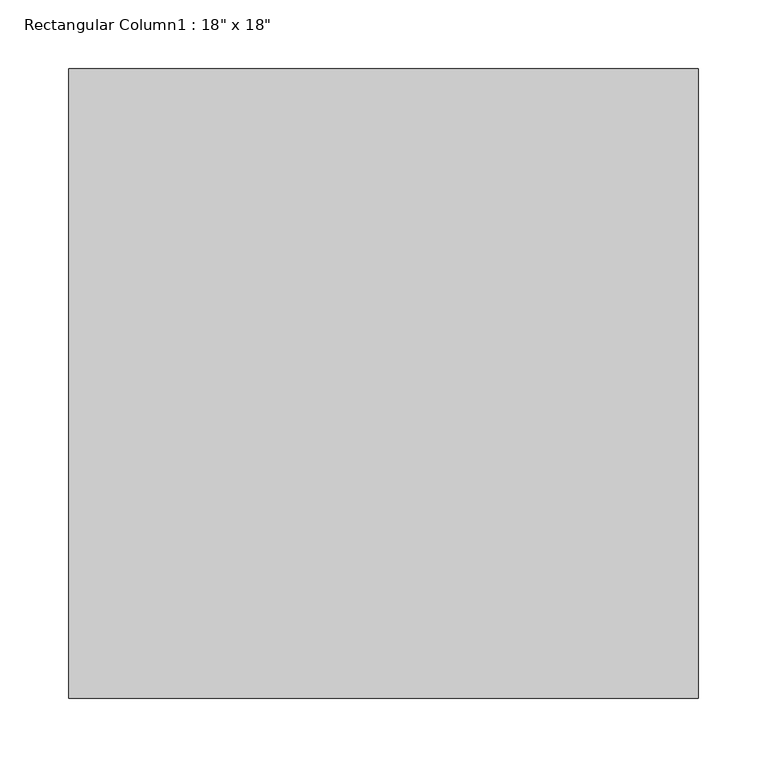
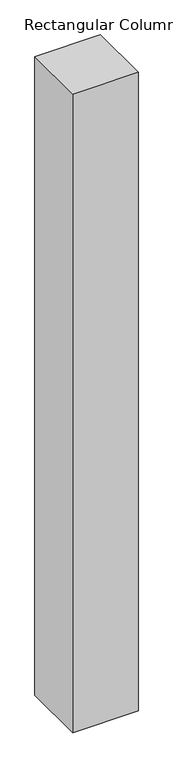
"""IFC4 building model written with IfcOpenShell, lengths in millimetres: column geometry."""

import ifcopenshell
import ifcopenshell.guid

model = None  # the IFC model being written
_history = None  # IfcOwnerHistory: only IFC2X3 demands one
_inside = {}  # id of a spatial element -> (the spatial element, [elements in it])
_under = {}  # id of a project, library or spatial element -> (it, [spatial elements below it])
_declared = {}  # id of a project -> (the project, [libraries it declares])
_typed = {}  # id of a type object -> (the type object, [elements of that type])
_made_of = {}  # id of a material, layer set ... -> (it, [elements and type objects made of it])


def new_model(schema):
    """Start an empty IFC model of exactly this schema.

    Asked for "IFC4X3", IfcOpenShell would pick the latest addendum, in which some entities
    have other attributes; the version numbers below select the first issue.
    IFC2X3 requires an IfcOwnerHistory on every rooted entity: one is made here for all.
    """
    global model, _history
    if schema == "IFC4X3":
        model = ifcopenshell.file(schema_version=(4, 3, 0, 0))
    else:
        model = ifcopenshell.file(schema=schema)
    _inside.clear()
    _under.clear()
    _declared.clear()
    _typed.clear()
    _made_of.clear()
    _history = None
    if model.schema == "IFC2X3":
        org = make("IfcOrganization", Name="unknown")
        user = make(
            "IfcPersonAndOrganization",
            ThePerson=make("IfcPerson", FamilyName="unknown"),
            TheOrganization=org,
        )
        app = make(
            "IfcApplication",
            ApplicationDeveloper=org,
            Version="unknown",
            ApplicationFullName="unknown",
            ApplicationIdentifier="unknown",
        )
        _history = make(
            "IfcOwnerHistory",
            OwningUser=user,
            OwningApplication=app,
            ChangeAction="ADDED",
            CreationDate=0,
        )
    return model


def make(cls, **values):
    """One entity of the class cls with the attributes given. An attribute that is None is left unset."""
    return model.create_entity(
        cls, **{name: value for name, value in values.items() if value is not None}
    )


def rooted(cls, **values):
    """An entity with a GlobalId (a new one), such as an element, a storey or a relation."""
    return make(cls, GlobalId=ifcopenshell.guid.new(), OwnerHistory=_history, **values)


def si_unit(unit_type, name, prefix=None):
    """IfcSIUnit, for example si_unit("LENGTHUNIT", "METRE", prefix="MILLI")."""
    return make("IfcSIUnit", UnitType=unit_type, Prefix=prefix, Name=name)


def assignment(units):
    """IfcUnitAssignment: the units of a project."""
    return None if units is None else make("IfcUnitAssignment", Units=units)


def point(xyz):
    """IfcCartesianPoint."""
    return None if xyz is None else make("IfcCartesianPoint", Coordinates=xyz)


def direction(xyz):
    """IfcDirection."""
    return None if xyz is None else make("IfcDirection", DirectionRatios=xyz)


def frame(location, z_axis=None, x_axis=None):
    """IfcAxis2Placement3D, a coordinate frame: its origin and axes. An axis left out is left unset."""
    return make(
        "IfcAxis2Placement3D",
        Location=point(location),
        Axis=direction(z_axis),
        RefDirection=direction(x_axis),
    )


def origin():
    """The frame at (0, 0, 0) with its axes left unset."""
    return frame((0.0, 0.0, 0.0))


def place(relative_to, where):
    """IfcLocalPlacement: puts the frame where relative to a parent placement (None: the world)."""
    return make(
        "IfcLocalPlacement", PlacementRelTo=relative_to, RelativePlacement=where
    )


def context(
    kind, dimensions, precision=None, world=None, true_north=None, identifier=None
):
    """IfcGeometricRepresentationContext, for example the 3D "Model" context."""
    return make(
        "IfcGeometricRepresentationContext",
        ContextIdentifier=identifier,
        ContextType=kind,
        CoordinateSpaceDimension=dimensions,
        Precision=precision,
        WorldCoordinateSystem=world,
        TrueNorth=true_north,
    )


def project(units=None, contexts=None):
    """IfcProject with its units and contexts."""
    return rooted(
        "IfcProject",
        Name="project",
        RepresentationContexts=contexts,
        UnitsInContext=assignment(units),
    )


def spatial(cls, under=None, at=None, **own):
    """A site, building, storey or space (cls), placed at a placement, below another one or the project."""
    s = rooted(cls, ObjectPlacement=at, **own)
    if under is not None:
        _under.setdefault(under.id(), (under, []))[1].append(s)
    return s


def polyline(points):
    """IfcPolyline through the points."""
    return make("IfcPolyline", Points=[point(p) for p in points])


def outline(outer, holes=None, kind="AREA"):
    """IfcArbitraryClosedProfileDef: a profile drawn as a closed curve; with holes, ...WithVoids."""
    if holes is None:
        return make("IfcArbitraryClosedProfileDef", ProfileType=kind, OuterCurve=outer)
    return make(
        "IfcArbitraryProfileDefWithVoids",
        ProfileType=kind,
        OuterCurve=outer,
        InnerCurves=holes,
    )


def extrude(swept, where, along, depth):
    """IfcExtrudedAreaSolid: the profile swept, set in the frame where, extruded along a direction by depth."""
    return make(
        "IfcExtrudedAreaSolid",
        SweptArea=swept,
        Position=where,
        ExtrudedDirection=direction(along),
        Depth=depth,
    )


def shape(context_of_items, identifier, shape_type, items):
    """IfcShapeRepresentation: the items that make up one representation, for example the "Body"."""
    return make(
        "IfcShapeRepresentation",
        ContextOfItems=context_of_items,
        RepresentationIdentifier=identifier,
        RepresentationType=shape_type,
        Items=items,
    )


def source(mapping_origin, context_of_items, identifier, shape_type, items):
    """IfcRepresentationMap: a shape defined once, which mapped items show again and again."""
    return make(
        "IfcRepresentationMap",
        MappingOrigin=mapping_origin,
        MappedRepresentation=shape(context_of_items, identifier, shape_type, items),
    )


def transform(
    local_origin,
    x_axis=None,
    y_axis=None,
    z_axis=None,
    scale=None,
    scale2=None,
    scale3=None,
    uniform=True,
):
    """IfcCartesianTransformationOperator3D, or its non-uniform kind. x_axis, y_axis, z_axis: its Axis1, 2, 3."""
    if uniform:
        return make(
            "IfcCartesianTransformationOperator3D",
            Axis1=direction(x_axis),
            Axis2=direction(y_axis),
            LocalOrigin=point(local_origin),
            Scale=scale,
            Axis3=direction(z_axis),
        )
    return make(
        "IfcCartesianTransformationOperator3DnonUniform",
        Axis1=direction(x_axis),
        Axis2=direction(y_axis),
        LocalOrigin=point(local_origin),
        Scale=scale,
        Axis3=direction(z_axis),
        Scale2=scale2,
        Scale3=scale3,
    )


def mapped(mapping_source, mapping_target):
    """IfcMappedItem: shows the shape of a source again, moved by a transform."""
    return make(
        "IfcMappedItem", MappingSource=mapping_source, MappingTarget=mapping_target
    )


def made_of(thing, what):
    """Note that an element or type object is made of a material, layer set ...; save() writes the relation."""
    if what is not None:
        _made_of.setdefault(what.id(), (what, []))[1].append(thing)
    return thing


def element(
    cls,
    number,
    at=None,
    inside=None,
    cuts=None,
    type_object=None,
    material=None,
    context=None,
    identifier="Body",
    shape_type=None,
    held_by="IfcProductDefinitionShape",
    body=None,
    shapes=None,
    **own,
):
    """One element of the class cls, such as IfcWall. Its Tag is "e" and its number.

    at: its placement. inside: the storey or other place that contains it. cuts: it is an
    opening in that element (IfcRelVoidsElement). A single representation is given by context,
    identifier, shape_type and body (its items); several are given by shapes. held_by: the class
    of the entity that holds the representations. save() writes the other relations.
    """
    e = rooted(cls, Tag="e%d" % number, ObjectPlacement=at, **own)
    if body is not None:
        shapes = [shape(context, identifier, shape_type, body)]
    if shapes is not None:
        e.Representation = make(held_by, Representations=shapes)
    if inside is not None:
        _inside.setdefault(inside.id(), (inside, []))[1].append(e)
    if cuts is not None:
        rooted(
            "IfcRelVoidsElement", RelatingBuildingElement=cuts, RelatedOpeningElement=e
        )
    if type_object is not None:
        _typed.setdefault(type_object.id(), (type_object, []))[1].append(e)
    return made_of(e, material)


def aggregate(whole, parts):
    """IfcRelAggregates: a whole, such as a stair, and the parts it consists of."""
    return rooted("IfcRelAggregates", RelatingObject=whole, RelatedObjects=parts)


def save(model, path):
    """Write the relations noted so far, then the file.

    IfcRelAggregates (storeys below a building ...), IfcRelContainedInSpatialStructure (elements
    in a storey), IfcRelDefinesByType, IfcRelAssociatesMaterial and IfcRelDeclares: one each for
    every whole, place, type object, material and project.
    """
    for whole, parts in _under.values():
        aggregate(whole, parts)
    for where, things in _inside.values():
        rooted(
            "IfcRelContainedInSpatialStructure",
            RelatedElements=things,
            RelatingStructure=where,
        )
    for kind, things in _typed.values():
        rooted("IfcRelDefinesByType", RelatedObjects=things, RelatingType=kind)
    for what, things in _made_of.values():
        rooted("IfcRelAssociatesMaterial", RelatedObjects=things, RelatingMaterial=what)
    for by, libraries in _declared.values():
        rooted("IfcRelDeclares", RelatingContext=by, RelatedDefinitions=libraries)
    model.write(path)


def column_773d994b(model_context):
    return source(origin(), model_context, "Body", "SweptSolid", [
        extrude(outline(polyline([(228.6, 228.6), (228.6, -228.6), (-228.6, -228.6), (-228.6, 228.6), (228.6, 228.6)])), frame((0.0, 0.0, 14935.2), z_axis=(0.0, 0.0, 1.0), x_axis=(1.0, 0.0, 0.0)), (0.0, 0.0, 1.0), 4724.4),
    ])


if __name__ == "__main__":
    model = new_model("IFC4")
    model_context = context("Model", 3, world=origin())
    ifc_project = project(units=[si_unit("LENGTHUNIT", "METRE", prefix="MILLI")], contexts=[model_context])
    site = spatial("IfcSite", under=ifc_project)
    building = spatial("IfcBuilding", under=site)
    placement = place(None, origin())
    column_shape = column_773d994b(model_context)
    element("IfcColumn", 1, ObjectType="Rectangular Column1 : 18\" x 18\"", at=placement, inside=building, context=model_context, shape_type="MappedRepresentation", body=[
        mapped(column_shape, transform((0.0, 0.0, 0.0), x_axis=(1.0, 0.0, 0.0), y_axis=(0.0, 1.0, 0.0), z_axis=(0.0, 0.0, 1.0))),
    ])
    save(model, "model.ifc")

# Revit data of these elements
# Type "Rectangular Column1 : 18\" x 18\""
#   Depth = 1' - 6"
#   Width = 1' - 6"
